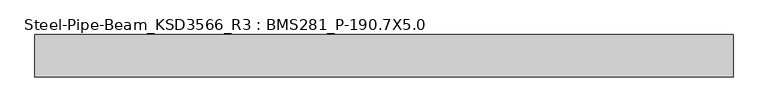
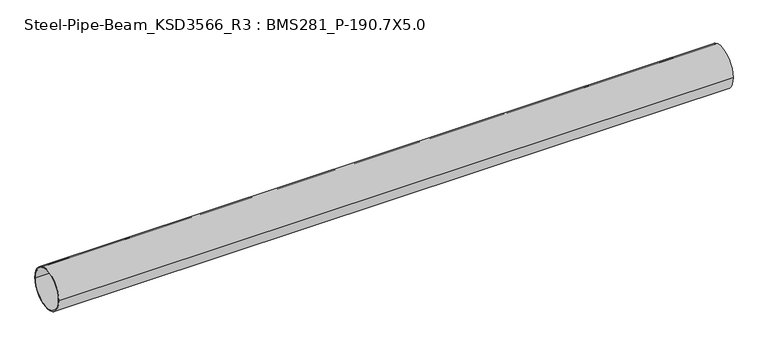
"""IFC4 building model written with IfcOpenShell, lengths in millimetres: member geometry, Steel-Pipe-Beam_KSD3566_R3 : BMS281_P-190.7X5.0."""

from ifc_helpers import new_model, si_unit, point, frame, origin, origin_2d, place, context, project, spatial, circle_curve, trimmed, segment, composite_curve, outline, extrude, source, transform, mapped, element, save


def steel_pipe_beam_ksd3566_r3_bms281_p_190_7x5_0_547b39ae(model_context):
    return source(origin(), model_context, "Body", "SweptSolid", [
        extrude(outline(composite_curve([segment(trimmed(circle_curve(origin_2d(), 95.35), [point((-95.35, 0.0))], [point((95.35, 0.0))], False, "CARTESIAN"), True, "CONTINUOUS"), segment(trimmed(circle_curve(origin_2d(), 95.35), [point((95.35, 0.0))], [point((-95.35, 0.0))], False, "CARTESIAN"), True, "CONTINUOUS")], self_intersect=False), holes=[composite_curve([segment(trimmed(circle_curve(origin_2d(), 90.35), [point((90.35, 0.0))], [point((-90.35, 0.0))], True, "CARTESIAN"), True, "CONTINUOUS"), segment(trimmed(circle_curve(origin_2d(), 90.35), [point((-90.35, 0.0))], [point((90.35, 0.0))], True, "CARTESIAN"), True, "CONTINUOUS")], self_intersect=False)]), frame((-1617.156438, 0.0, 0.0), z_axis=(1.0, 0.0, 0.0), x_axis=(0.0, 1.0, 0.0)), (0.0, 0.0, 1.0), 3133.1971631),
    ])


if __name__ == "__main__":
    model = new_model("IFC4")
    model_context = context("Model", 3, world=origin())
    ifc_project = project(units=[si_unit("LENGTHUNIT", "METRE", prefix="MILLI")], contexts=[model_context])
    site = spatial("IfcSite", under=ifc_project)
    building = spatial("IfcBuilding", under=site)
    placement = place(None, origin())
    steel_pipe_beam_ksd3566_r3_bms281_p_190_7x5_0_shape = steel_pipe_beam_ksd3566_r3_bms281_p_190_7x5_0_547b39ae(model_context)
    element("IfcMember", 1, ObjectType="Steel-Pipe-Beam_KSD3566_R3 : BMS281_P-190.7X5.0", at=placement, inside=building, context=model_context, shape_type="MappedRepresentation", body=[
        mapped(steel_pipe_beam_ksd3566_r3_bms281_p_190_7x5_0_shape, transform((0.0, 0.0, 0.0), x_axis=(1.0, 0.0, 0.0), y_axis=(0.0, 1.0, 0.0), z_axis=(0.0, 0.0, 1.0))),
    ])
    save(model, "model.ifc")

# Revit data of these elements
# Type "Steel-Pipe-Beam_KSD3566_R3 : BMS281_P-190.7X5.0"
#   Keynote = "P-190.7X5.0"
#   SteelWeight = "Light"
#   t = 0.0050 m
#   Surface Area = 0.599102 m²/m
#   Section Area = 29.1697 cm²
#   Mass per Unit Length = 22.8982 kg/m
#   Length [instance default] = 1.5000 m
#   D = 0.1907 m
#   hec_material4 [instance default] = none
#   hec_material3 [instance default] = none
#   hec_material2 [instance default] = none
#   hec_material1 [instance default] = none
#   Structural Material [instance default] = Steel, 45-345
#   Assembly Code = ""
# Element 1 (IfcMember, "Steel-Pipe-Beam_KSD3566_R3 : BMS281_P-190.7X5.0")
#   Structural Material = none
# Materials
#   "Steel, 45-345": class "Metal", colour RGB 189 187 185, transparency 0, Description = "Steel 345 MPa", Cost = 0
